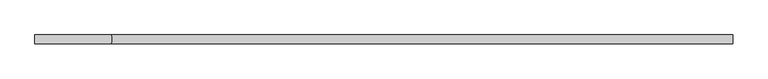
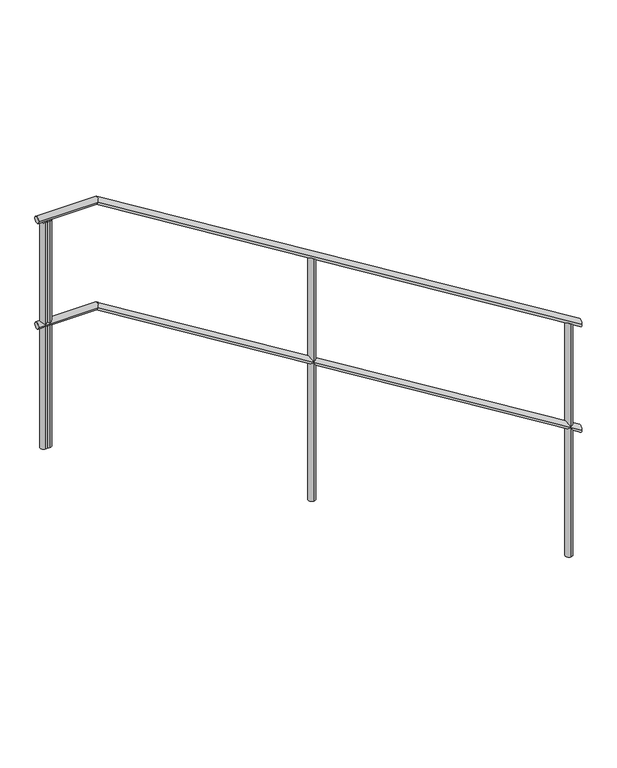
"""IFC4 building model written with IfcOpenShell, lengths in millimetres: railing geometry."""

from ifc_helpers import new_model, si_unit, point, frame, frame_2d, origin, place, context, project, spatial, circle_curve, ellipse_curve, trimmed, segment, composite_curve, outline, extrude, source, transform, mapped, element, save
from ifc_brep_helpers import plane_surface, cylinder_surface, advanced_brep


def railing_090315b5(model_context):
    return source(origin(), model_context, "Body", "SolidModel", [
        advanced_brep(
        [(28470.0, -4687.9791411, -450.9609787), (28470.0, -4717.9791411, -450.9609787), (26305.7432145, -4687.9791411, 885.0), (26305.7432145, -4717.9791411, 885.0), (26040.0, -4687.9791411, 885.0), (26040.0, -4717.9791411, 885.0)],
        [
            (0, 1, ellipse_curve(frame((28470.0, -4702.9791411, -450.9609787), z_axis=(1.0, 0.0, 0.0), x_axis=(0.0, 0.0, -1.0)), 17.6276454, 15.0)),
            (1, 0, ellipse_curve(frame((28470.0, -4702.9791411, -450.9609787), z_axis=(1.0, 0.0, 0.0), x_axis=(0.0, 0.0, -1.0)), 17.6276454, 15.0)),
            (0, 2),
            (2, 3, ellipse_curve(frame((26305.7432145, -4702.9791411, 885.0), z_axis=(0.9620125025549409, 0.0, -0.27300539358770864), x_axis=(-0.27300539358770803, 0.0, -0.9620125025549412)), 15.5923129, 15.0)),
            (3, 1),
            (3, 2, ellipse_curve(frame((26305.7432145, -4702.9791411, 885.0), z_axis=(0.9620125025549409, 0.0, -0.27300539358770864), x_axis=(-0.27300539358770803, 0.0, -0.9620125025549412)), 15.5923129, 15.0)),
            (4, 5, circle_curve(frame((26040.0, -4702.9791411, 885.0), z_axis=(-1.0, 0.0, 0.0), x_axis=(0.0, -1.0, 0.0)), 15.0)),
            (5, 4, circle_curve(frame((26040.0, -4702.9791411, 885.0), z_axis=(-1.0, 0.0, 0.0), x_axis=(0.0, -1.0, 0.0)), 15.0)),
            (2, 4),
            (5, 3),
        ],
        [
            plane_surface(frame((28470.0, -4702.9791411, -433.3333333), z_axis=(1.0, 0.0, 0.0), x_axis=(0.0, -1.0, 0.0))),
            cylinder_surface(frame((28462.1209619, -4702.9791411, -446.097375), z_axis=(0.8509361101440404, 0.0, -0.5252692037926168), x_axis=(0.0, -1.0, 0.0)), 15.0),
            plane_surface(frame((26040.0, -4702.9791411, 900.0), z_axis=(-1.0, 0.0, 0.0), x_axis=(0.0, -1.0, 0.0))),
            cylinder_surface(frame((26310.0, -4702.9791411, 885.0), z_axis=(1.0, 0.0, 0.0), x_axis=(0.0, -1.0, 0.0)), 15.0),
        ],
        [
            (0, [[1, 2]]),
            (1, [[-1, 3, 4, 5]]),
            (1, [[-2, -5, 6, -3]]),
            (2, [[7, 8]]),
            (3, [[-4, 9, -8, 10]]),
            (3, [[-6, -10, -7, -9]]),
        ],
    ),
        advanced_brep(
        [(28470.0, -4687.9791411, 49.0390213), (28470.0, -4717.9791411, 49.0390213), (26305.7432145, -4687.9791411, 1385.0), (26305.7432145, -4717.9791411, 1385.0), (26040.0, -4687.9791411, 1385.0), (26040.0, -4717.9791411, 1385.0)],
        [
            (0, 1, ellipse_curve(frame((28470.0, -4702.9791411, 49.0390213), z_axis=(1.0, 0.0, 0.0), x_axis=(0.0, 0.0, -1.0)), 17.6276454, 15.0)),
            (1, 0, ellipse_curve(frame((28470.0, -4702.9791411, 49.0390213), z_axis=(1.0, 0.0, 0.0), x_axis=(0.0, 0.0, -1.0)), 17.6276454, 15.0)),
            (0, 2),
            (2, 3, ellipse_curve(frame((26305.7432145, -4702.9791411, 1385.0), z_axis=(0.9620125025549409, 0.0, -0.27300539358770864), x_axis=(-0.27300539358770803, 0.0, -0.9620125025549412)), 15.5923129, 15.0)),
            (3, 1),
            (3, 2, ellipse_curve(frame((26305.7432145, -4702.9791411, 1385.0), z_axis=(0.9620125025549409, 0.0, -0.27300539358770864), x_axis=(-0.27300539358770803, 0.0, -0.9620125025549412)), 15.5923129, 15.0)),
            (4, 5, circle_curve(frame((26040.0, -4702.9791411, 1385.0), z_axis=(-1.0, 0.0, 0.0), x_axis=(0.0, -1.0, 0.0)), 15.0)),
            (5, 4, circle_curve(frame((26040.0, -4702.9791411, 1385.0), z_axis=(-1.0, 0.0, 0.0), x_axis=(0.0, -1.0, 0.0)), 15.0)),
            (2, 4),
            (5, 3),
        ],
        [
            plane_surface(frame((28470.0, -4702.9791411, 66.6666667), z_axis=(1.0, 0.0, 0.0), x_axis=(0.0, -1.0, 0.0))),
            cylinder_surface(frame((28462.1209619, -4702.9791411, 53.902625), z_axis=(0.8509361101440404, 0.0, -0.5252692037926168), x_axis=(0.0, -1.0, 0.0)), 15.0),
            plane_surface(frame((26040.0, -4702.9791411, 1400.0), z_axis=(-1.0, 0.0, 0.0), x_axis=(0.0, -1.0, 0.0))),
            cylinder_surface(frame((26310.0, -4702.9791411, 1385.0), z_axis=(1.0, 0.0, 0.0), x_axis=(0.0, -1.0, 0.0)), 15.0),
        ],
        [
            (0, [[1, 2]]),
            (1, [[-1, 3, 4, 5]]),
            (1, [[-2, -5, 6, -3]]),
            (2, [[7, 8]]),
            (3, [[-4, 9, -8, 10]]),
            (3, [[-6, -10, -7, -9]]),
        ],
    ),
        extrude(outline(composite_curve([segment(trimmed(circle_curve(frame_2d((26070.0, -4702.9791411)), 15.0), [point((26070.0, -4687.9791411))], [point((26070.0, -4717.9791411))], False, "CARTESIAN"), True, "CONTINUOUS"), segment(trimmed(circle_curve(frame_2d((26070.0, -4702.9791411)), 15.0), [point((26070.0, -4717.9791411))], [point((26070.0, -4687.9791411))], False, "CARTESIAN"), True, "CONTINUOUS")], self_intersect=False)), frame((0.0, 0.0, 300.0), z_axis=(0.0, 0.0, 1.0), x_axis=(1.0, 0.0, 0.0)), (0.0, 0.0, 1.0), 1070.0),
        advanced_brep(
        [(27270.0, -4717.9791411, 777.4074074), (27270.0, -4687.9791411, 777.4074074), (27270.0, -4687.9791411, -366.6666667), (27270.0, -4717.9791411, -366.6666667)],
        [
            (0, 1, ellipse_curve(frame((27270.0, -4702.9791411, 777.4074074), z_axis=(-0.5252692037926167, 0.0, -0.8509361101440406), x_axis=(-0.8509361101440406, 0.0, 0.5252692037926162)), 17.6276454, 15.0)),
            (1, 2),
            (2, 3, circle_curve(frame((27270.0, -4702.9791411, -366.6666667), z_axis=(0.0, 0.0, 1.0), x_axis=(0.0, 1.0, 0.0)), 15.0)),
            (3, 0),
            (3, 2, circle_curve(frame((27270.0, -4702.9791411, -366.6666667), z_axis=(0.0, 0.0, 1.0), x_axis=(0.0, 1.0, 0.0)), 15.0)),
            (1, 0, ellipse_curve(frame((27270.0, -4702.9791411, 777.4074074), z_axis=(-0.5252692037926167, 0.0, -0.8509361101440406), x_axis=(-0.8509361101440406, 0.0, 0.5252692037926162)), 17.6276454, 15.0)),
        ],
        [
            cylinder_surface(frame((27270.0, -4702.9791411, -466.6666667), z_axis=(0.0, 0.0, 1.0), x_axis=(0.0, 1.0, 0.0)), 15.0),
            plane_surface(frame((27245.0, -4677.9791411, 792.8395062), z_axis=(0.5252692037926167, 0.0, 0.8509361101440406), x_axis=(0.0, -1.0, 0.0))),
            plane_surface(frame((27295.0, -4677.9791411, -366.6666667), z_axis=(0.0, 0.0, -1.0), x_axis=(0.0, -1.0, 0.0))),
        ],
        [
            (0, [[1, 2, 3, 4]]),
            (0, [[5, -2, 6, -4]]),
            (1, [[-6, -1]]),
            (2, [[-5, -3]]),
        ],
    ),
        extrude(outline(composite_curve([segment(trimmed(circle_curve(frame_2d((26090.0, -4702.9791411)), 15.0), [point((26090.0, -4687.9791411))], [point((26090.0, -4717.9791411))], False, "CARTESIAN"), True, "CONTINUOUS"), segment(trimmed(circle_curve(frame_2d((26090.0, -4702.9791411)), 15.0), [point((26090.0, -4717.9791411))], [point((26090.0, -4687.9791411))], False, "CARTESIAN"), True, "CONTINUOUS")], self_intersect=False)), frame((0.0, 0.0, 300.0), z_axis=(0.0, 0.0, 1.0), x_axis=(1.0, 0.0, 0.0)), (0.0, 0.0, 1.0), 1070.0),
        advanced_brep(
        [(28420.0, -4717.9791411, 67.5308642), (28420.0, -4687.9791411, 67.5308642), (28420.0, -4687.9791411, -1033.3333333), (28420.0, -4717.9791411, -1033.3333333)],
        [
            (0, 1, ellipse_curve(frame((28420.0, -4702.9791411, 67.5308642), z_axis=(-0.5252692037926167, 0.0, -0.8509361101440406), x_axis=(-0.8509361101440406, 0.0, 0.5252692037926162)), 17.6276454, 15.0)),
            (1, 2),
            (2, 3, circle_curve(frame((28420.0, -4702.9791411, -1033.3333333), z_axis=(0.0, 0.0, 1.0), x_axis=(0.0, 1.0, 0.0)), 15.0)),
            (3, 0),
            (3, 2, circle_curve(frame((28420.0, -4702.9791411, -1033.3333333), z_axis=(0.0, 0.0, 1.0), x_axis=(0.0, 1.0, 0.0)), 15.0)),
            (1, 0, ellipse_curve(frame((28420.0, -4702.9791411, 67.5308642), z_axis=(-0.5252692037926167, 0.0, -0.8509361101440406), x_axis=(-0.8509361101440406, 0.0, 0.5252692037926162)), 17.6276454, 15.0)),
        ],
        [
            cylinder_surface(frame((28420.0, -4702.9791411, -1133.3333333), z_axis=(0.0, 0.0, 1.0), x_axis=(0.0, 1.0, 0.0)), 15.0),
            plane_surface(frame((28395.0, -4677.9791411, 82.962963), z_axis=(0.5252692037926167, 0.0, 0.8509361101440406), x_axis=(0.0, -1.0, 0.0))),
            plane_surface(frame((28445.0, -4677.9791411, -1033.3333333), z_axis=(0.0, 0.0, -1.0), x_axis=(0.0, -1.0, 0.0))),
        ],
        [
            (0, [[1, 2, 3, 4]]),
            (0, [[5, -2, 6, -4]]),
            (1, [[-6, -1]]),
            (2, [[-5, -3]]),
        ],
    ),
    ])


if __name__ == "__main__":
    model = new_model("IFC4")
    model_context = context("Model", 3, world=origin())
    ifc_project = project(units=[si_unit("LENGTHUNIT", "METRE", prefix="MILLI")], contexts=[model_context])
    site = spatial("IfcSite", under=ifc_project)
    building = spatial("IfcBuilding", under=site)
    placement = place(None, origin())
    railing_shape = railing_090315b5(model_context)
    element("IfcRailing", 1, at=placement, inside=building, context=model_context, shape_type="MappedRepresentation", body=[
        mapped(railing_shape, transform((0.0, 0.0, 0.0), x_axis=(1.0, 0.0, 0.0), y_axis=(0.0, 1.0, 0.0), z_axis=(0.0, 0.0, 1.0))),
    ])
    save(model, "model.ifc")
